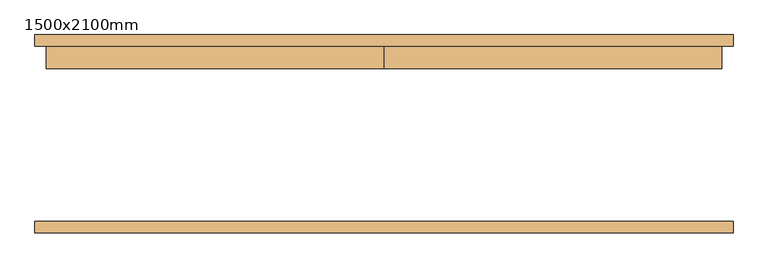
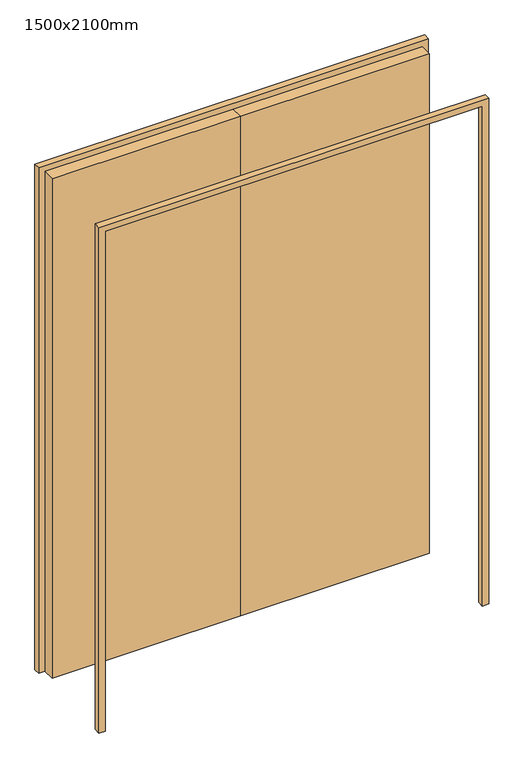
"""IFC4 building model written with IfcOpenShell, lengths in millimetres: door geometry, WWm-DoubleSolid-Flush : 1500x2100mm."""

import ifcopenshell
import ifcopenshell.guid

model = None  # the IFC model being written
_history = None  # IfcOwnerHistory: only IFC2X3 demands one
_inside = {}  # id of a spatial element -> (the spatial element, [elements in it])
_under = {}  # id of a project, library or spatial element -> (it, [spatial elements below it])
_declared = {}  # id of a project -> (the project, [libraries it declares])
_typed = {}  # id of a type object -> (the type object, [elements of that type])
_made_of = {}  # id of a material, layer set ... -> (it, [elements and type objects made of it])


def new_model(schema):
    """Start an empty IFC model of exactly this schema.

    Asked for "IFC4X3", IfcOpenShell would pick the latest addendum, in which some entities
    have other attributes; the version numbers below select the first issue.
    IFC2X3 requires an IfcOwnerHistory on every rooted entity: one is made here for all.
    """
    global model, _history
    if schema == "IFC4X3":
        model = ifcopenshell.file(schema_version=(4, 3, 0, 0))
    else:
        model = ifcopenshell.file(schema=schema)
    _inside.clear()
    _under.clear()
    _declared.clear()
    _typed.clear()
    _made_of.clear()
    _history = None
    if model.schema == "IFC2X3":
        org = make("IfcOrganization", Name="unknown")
        user = make(
            "IfcPersonAndOrganization",
            ThePerson=make("IfcPerson", FamilyName="unknown"),
            TheOrganization=org,
        )
        app = make(
            "IfcApplication",
            ApplicationDeveloper=org,
            Version="unknown",
            ApplicationFullName="unknown",
            ApplicationIdentifier="unknown",
        )
        _history = make(
            "IfcOwnerHistory",
            OwningUser=user,
            OwningApplication=app,
            ChangeAction="ADDED",
            CreationDate=0,
        )
    return model


def make(cls, **values):
    """One entity of the class cls with the attributes given. An attribute that is None is left unset."""
    return model.create_entity(
        cls, **{name: value for name, value in values.items() if value is not None}
    )


def rooted(cls, **values):
    """An entity with a GlobalId (a new one), such as an element, a storey or a relation."""
    return make(cls, GlobalId=ifcopenshell.guid.new(), OwnerHistory=_history, **values)


def si_unit(unit_type, name, prefix=None):
    """IfcSIUnit, for example si_unit("LENGTHUNIT", "METRE", prefix="MILLI")."""
    return make("IfcSIUnit", UnitType=unit_type, Prefix=prefix, Name=name)


def assignment(units):
    """IfcUnitAssignment: the units of a project."""
    return None if units is None else make("IfcUnitAssignment", Units=units)


def point(xyz):
    """IfcCartesianPoint."""
    return None if xyz is None else make("IfcCartesianPoint", Coordinates=xyz)


def direction(xyz):
    """IfcDirection."""
    return None if xyz is None else make("IfcDirection", DirectionRatios=xyz)


def frame(location, z_axis=None, x_axis=None):
    """IfcAxis2Placement3D, a coordinate frame: its origin and axes. An axis left out is left unset."""
    return make(
        "IfcAxis2Placement3D",
        Location=point(location),
        Axis=direction(z_axis),
        RefDirection=direction(x_axis),
    )


def origin():
    """The frame at (0, 0, 0) with its axes left unset."""
    return frame((0.0, 0.0, 0.0))


def origin_with_axes():
    """The frame at (0, 0, 0) with the z axis (0, 0, 1) and the x axis (1, 0, 0) written out."""
    return frame((0.0, 0.0, 0.0), z_axis=(0.0, 0.0, 1.0), x_axis=(1.0, 0.0, 0.0))


def place(relative_to, where):
    """IfcLocalPlacement: puts the frame where relative to a parent placement (None: the world)."""
    return make(
        "IfcLocalPlacement", PlacementRelTo=relative_to, RelativePlacement=where
    )


def context(
    kind, dimensions, precision=None, world=None, true_north=None, identifier=None
):
    """IfcGeometricRepresentationContext, for example the 3D "Model" context."""
    return make(
        "IfcGeometricRepresentationContext",
        ContextIdentifier=identifier,
        ContextType=kind,
        CoordinateSpaceDimension=dimensions,
        Precision=precision,
        WorldCoordinateSystem=world,
        TrueNorth=true_north,
    )


def project(units=None, contexts=None):
    """IfcProject with its units and contexts."""
    return rooted(
        "IfcProject",
        Name="project",
        RepresentationContexts=contexts,
        UnitsInContext=assignment(units),
    )


def spatial(cls, under=None, at=None, **own):
    """A site, building, storey or space (cls), placed at a placement, below another one or the project."""
    s = rooted(cls, ObjectPlacement=at, **own)
    if under is not None:
        _under.setdefault(under.id(), (under, []))[1].append(s)
    return s


def polyline(points):
    """IfcPolyline through the points."""
    return make("IfcPolyline", Points=[point(p) for p in points])


def outline(outer, holes=None, kind="AREA"):
    """IfcArbitraryClosedProfileDef: a profile drawn as a closed curve; with holes, ...WithVoids."""
    if holes is None:
        return make("IfcArbitraryClosedProfileDef", ProfileType=kind, OuterCurve=outer)
    return make(
        "IfcArbitraryProfileDefWithVoids",
        ProfileType=kind,
        OuterCurve=outer,
        InnerCurves=holes,
    )


def extrude(swept, where, along, depth):
    """IfcExtrudedAreaSolid: the profile swept, set in the frame where, extruded along a direction by depth."""
    return make(
        "IfcExtrudedAreaSolid",
        SweptArea=swept,
        Position=where,
        ExtrudedDirection=direction(along),
        Depth=depth,
    )


def shape(context_of_items, identifier, shape_type, items):
    """IfcShapeRepresentation: the items that make up one representation, for example the "Body"."""
    return make(
        "IfcShapeRepresentation",
        ContextOfItems=context_of_items,
        RepresentationIdentifier=identifier,
        RepresentationType=shape_type,
        Items=items,
    )


def source(mapping_origin, context_of_items, identifier, shape_type, items):
    """IfcRepresentationMap: a shape defined once, which mapped items show again and again."""
    return make(
        "IfcRepresentationMap",
        MappingOrigin=mapping_origin,
        MappedRepresentation=shape(context_of_items, identifier, shape_type, items),
    )


def transform(
    local_origin,
    x_axis=None,
    y_axis=None,
    z_axis=None,
    scale=None,
    scale2=None,
    scale3=None,
    uniform=True,
):
    """IfcCartesianTransformationOperator3D, or its non-uniform kind. x_axis, y_axis, z_axis: its Axis1, 2, 3."""
    if uniform:
        return make(
            "IfcCartesianTransformationOperator3D",
            Axis1=direction(x_axis),
            Axis2=direction(y_axis),
            LocalOrigin=point(local_origin),
            Scale=scale,
            Axis3=direction(z_axis),
        )
    return make(
        "IfcCartesianTransformationOperator3DnonUniform",
        Axis1=direction(x_axis),
        Axis2=direction(y_axis),
        LocalOrigin=point(local_origin),
        Scale=scale,
        Axis3=direction(z_axis),
        Scale2=scale2,
        Scale3=scale3,
    )


def mapped(mapping_source, mapping_target):
    """IfcMappedItem: shows the shape of a source again, moved by a transform."""
    return make(
        "IfcMappedItem", MappingSource=mapping_source, MappingTarget=mapping_target
    )


def made_of(thing, what):
    """Note that an element or type object is made of a material, layer set ...; save() writes the relation."""
    if what is not None:
        _made_of.setdefault(what.id(), (what, []))[1].append(thing)
    return thing


def element(
    cls,
    number,
    at=None,
    inside=None,
    cuts=None,
    type_object=None,
    material=None,
    context=None,
    identifier="Body",
    shape_type=None,
    held_by="IfcProductDefinitionShape",
    body=None,
    shapes=None,
    **own,
):
    """One element of the class cls, such as IfcWall. Its Tag is "e" and its number.

    at: its placement. inside: the storey or other place that contains it. cuts: it is an
    opening in that element (IfcRelVoidsElement). A single representation is given by context,
    identifier, shape_type and body (its items); several are given by shapes. held_by: the class
    of the entity that holds the representations. save() writes the other relations.
    """
    e = rooted(cls, Tag="e%d" % number, ObjectPlacement=at, **own)
    if body is not None:
        shapes = [shape(context, identifier, shape_type, body)]
    if shapes is not None:
        e.Representation = make(held_by, Representations=shapes)
    if inside is not None:
        _inside.setdefault(inside.id(), (inside, []))[1].append(e)
    if cuts is not None:
        rooted(
            "IfcRelVoidsElement", RelatingBuildingElement=cuts, RelatedOpeningElement=e
        )
    if type_object is not None:
        _typed.setdefault(type_object.id(), (type_object, []))[1].append(e)
    return made_of(e, material)


def aggregate(whole, parts):
    """IfcRelAggregates: a whole, such as a stair, and the parts it consists of."""
    return rooted("IfcRelAggregates", RelatingObject=whole, RelatedObjects=parts)


def save(model, path):
    """Write the relations noted so far, then the file.

    IfcRelAggregates (storeys below a building ...), IfcRelContainedInSpatialStructure (elements
    in a storey), IfcRelDefinesByType, IfcRelAssociatesMaterial and IfcRelDeclares: one each for
    every whole, place, type object, material and project.
    """
    for whole, parts in _under.values():
        aggregate(whole, parts)
    for where, things in _inside.values():
        rooted(
            "IfcRelContainedInSpatialStructure",
            RelatedElements=things,
            RelatingStructure=where,
        )
    for kind, things in _typed.values():
        rooted("IfcRelDefinesByType", RelatedObjects=things, RelatingType=kind)
    for what, things in _made_of.values():
        rooted("IfcRelAssociatesMaterial", RelatedObjects=things, RelatingMaterial=what)
    for by, libraries in _declared.values():
        rooted("IfcRelDeclares", RelatingContext=by, RelatedDefinitions=libraries)
    model.write(path)


def door_1500x2100mm_1360b9d6(model_context):
    return source(origin(), model_context, "Body", "SweptSolid", [
        extrude(outline(polyline([(0.0, 195.0), (750.0, 195.0), (750.0, 145.0), (0.0, 145.0), (0.0, 195.0)])), origin_with_axes(), (0.0, 0.0, 1.0), 2100.0),
        extrude(outline(polyline([(-750.0, 195.0), (0.0, 195.0), (0.0, 145.0), (-750.0, 145.0), (-750.0, 195.0)])), origin_with_axes(), (0.0, 0.0, 1.0), 2100.0),
        extrude(outline(polyline([(2100.0, -750.0), (2100.0, 750.0), (0.0, 750.0), (0.0, 775.0), (2125.0, 775.0), (2125.0, -775.0), (0.0, -775.0), (0.0, -750.0), (2100.0, -750.0)])), frame((0.0, -220.0, 0.0), z_axis=(0.0, 1.0, 0.0), x_axis=(0.0, 0.0, 1.0)), (0.0, 0.0, 1.0), 25.0),
        extrude(outline(polyline([(2100.0, -750.0), (2100.0, 750.0), (0.0, 750.0), (0.0, 775.0), (2125.0, 775.0), (2125.0, -775.0), (0.0, -775.0), (0.0, -750.0), (2100.0, -750.0)])), frame((0.0, 195.0, 0.0), z_axis=(0.0, 1.0, 0.0), x_axis=(0.0, 0.0, 1.0)), (0.0, 0.0, 1.0), 25.0),
    ])


if __name__ == "__main__":
    model = new_model("IFC4")
    model_context = context("Model", 3, world=origin())
    ifc_project = project(units=[si_unit("LENGTHUNIT", "METRE", prefix="MILLI")], contexts=[model_context])
    site = spatial("IfcSite", under=ifc_project)
    building = spatial("IfcBuilding", under=site)
    placement = place(None, origin())
    door_1500x2100mm_shape = door_1500x2100mm_1360b9d6(model_context)
    element("IfcDoor", 1, ObjectType="WWm-DoubleSolid-Flush : 1500x2100mm", at=placement, inside=building, context=model_context, shape_type="MappedRepresentation", body=[
        mapped(door_1500x2100mm_shape, transform((0.0, 0.0, 0.0), x_axis=(1.0, 0.0, 0.0), y_axis=(0.0, 1.0, 0.0), z_axis=(0.0, 0.0, 1.0))),
    ])
    save(model, "model.ifc")

# Revit data of these elements
# Type "WWm-DoubleSolid-Flush : 1500x2100mm"
#   Type Mark = "EX1-56"
#   Construction Type Id = "MDOOR"
#   Assembly Code = "C1020"
#   Analytic Construction = "Metal"
#   Thickness = 50 mm
#   Thermal Resistance (R) = 0.270117 (m²·K)/W
#   Heat Transfer Coefficient (U) = 3.7021 W/(m²·K)
#   Height = 2100 mm
#   Trim Projection Ext = 25 mm
#   Trim Projection Int = 25 mm
#   Trim Width = 25 mm
#   Width = 1500 mm
#   Not 90 Degree [instance default] = no
#   90 Degree [instance default] = yes
#   Door Material = WW-EC-RGB-White
#   Frame Material = WW-EC-RGB-White
#   Visual Light Transmittance = 0
#   Solar Heat Gain Coefficient = 0
#   Function = (empty or 0)
#   Wall Closure = (empty or 0)
# Element 1 (IfcDoor, "WWm-DoubleSolid-Flush : 1500x2100mm")
#   Materials on its faces: "WW-EC-RGB-White"
# Materials
#   "WW-EC-RGB-White": class "Generic", colour RGB 255 255 255, transparency 0, Comments = "If region requests off-white, swith asset color to RGB 231-228-220", Description = "Generic Color", Cost = 0
